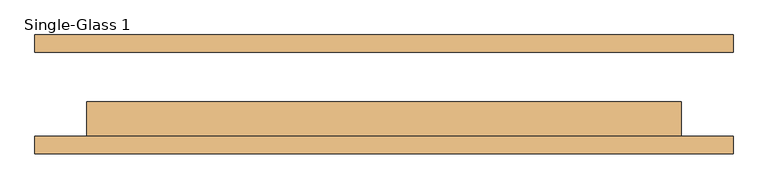
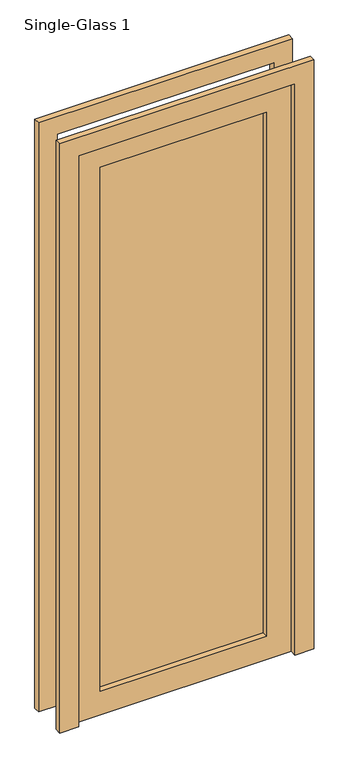
"""IFC4 building model written with IfcOpenShell, lengths in millimetres: door geometry, Single-Glass 1."""

from ifc_helpers import new_model, si_unit, frame, origin, place, context, project, spatial, polyline, outline, extrude, source, transform, mapped, element, save


def single_glass_1_9c89bfeb(model_context):
    return source(origin(), model_context, "Body", "SweptSolid", [
        extrude(outline(polyline([(2438.4, 437.35625), (0.0, 437.35625), (0.0, 513.55625), (2514.6, 513.55625), (2514.6, -513.55625), (0.0, -513.55625), (0.0, -437.35625), (2438.4, -437.35625), (2438.4, 437.35625)])), frame((0.0, 61.9125, 0.0), z_axis=(0.0, 1.0, 0.0), x_axis=(0.0, 0.0, 1.0)), (0.0, 0.0, 1.0), 25.4),
        extrude(outline(polyline([(2438.4, 437.35625), (0.0, 437.35625), (0.0, 513.55625), (2514.6, 513.55625), (2514.6, -513.55625), (0.0, -513.55625), (0.0, -437.35625), (2438.4, -437.35625), (2438.4, 437.35625)])), frame((0.0, -87.3125, 0.0), z_axis=(0.0, 1.0, 0.0), x_axis=(0.0, 0.0, 1.0)), (0.0, 0.0, 1.0), 25.4),
        extrude(outline(polyline([(335.75625, -33.3375), (335.75625, -39.6875), (-335.75625, -39.6875), (-335.75625, -33.3375), (335.75625, -33.3375)])), frame((0.0, 0.0, 101.6), z_axis=(0.0, 0.0, 1.0), x_axis=(1.0, 0.0, 0.0)), (0.0, 0.0, 1.0), 2235.2),
        extrude(outline(polyline([(2438.4, 437.35625), (2438.4, -437.35625), (0.0, -437.35625), (0.0, 437.35625), (2438.4, 437.35625)]), holes=[polyline([(2336.8, -335.75625), (2336.8, 335.75625), (101.6, 335.75625), (101.6, -335.75625), (2336.8, -335.75625)])]), frame((0.0, -61.9125, 0.0), z_axis=(0.0, 1.0, 0.0), x_axis=(0.0, 0.0, 1.0)), (0.0, 0.0, 1.0), 50.8),
    ])


if __name__ == "__main__":
    model = new_model("IFC4")
    model_context = context("Model", 3, world=origin())
    ifc_project = project(units=[si_unit("LENGTHUNIT", "METRE", prefix="MILLI")], contexts=[model_context])
    site = spatial("IfcSite", under=ifc_project)
    building = spatial("IfcBuilding", under=site)
    placement = place(None, origin())
    single_glass_1_shape = single_glass_1_9c89bfeb(model_context)
    element("IfcDoor", 1, ObjectType="Single-Glass 1 : 2'  10 7/16\" x96\"", at=placement, inside=building, context=model_context, shape_type="MappedRepresentation", body=[
        mapped(single_glass_1_shape, transform((0.0, 0.0, 0.0), x_axis=(1.0, 0.0, 0.0), y_axis=(0.0, 1.0, 0.0), z_axis=(0.0, 0.0, 1.0))),
    ])
    save(model, "model.ifc")

# Revit data of these elements
# Type "Single-Glass 1 : 2'  10 7/16\" x96\""
#   Type Mark = "41"
#   Construction Type Id = "MDOOR"
#   Assembly Code = "C1020"
#   Analytic Construction = "Metal"
#   Thickness = 0' - 2"
#   Heat Transfer Coefficient (U) = 3.7021 W/(m²·K)
#   Height = 8' - 0"
#   Rail Width - Base = 0' - 4"
#   Rail Width - Top = 0' - 4"
#   Stile Width - Hinge = 0' - 4"
#   Stile Width - Latch = 0' - 4"
#   Trim Projection Ext = 0' - 1"
#   Trim Projection Int = 0' - 1"
#   Trim Width = 0' - 3"
#   Width = 2' - 10 7/16"
#   Door Material = INTERIOR GRADE ALUMINUM STOREFRONT W/ SAFETY GLAZING
#   Frame Material = INTERIOR GRADE ALUMINUM STOREFRONT W/ SAFETY GLAZING
#   Visual Light Transmittance = 0
#   Solar Heat Gain Coefficient = 0
#   Function = (empty or 0)
#   Wall Closure = (empty or 0)
# Element 1 (IfcDoor, "Single-Glass 1 : 2'  10 7/16\" x96\"")
#   Materials on its faces: "INTERIOR GRADE ALUMINUM STOREFRONT W/ SAFETY GLAZING", "SAFETY GLAZING"
# Materials
#   "INTERIOR GRADE ALUMINUM STOREFRONT W/ SAFETY GLAZING": class "Metal", colour RGB 226 226 226, transparency 0, Description = "Aluminum 6061", Cost = 0
#   "SAFETY GLAZING": class "Glass", colour RGB 142 168 196, transparency 0.75, Description = "Soda Lime Glass", Cost = 0
